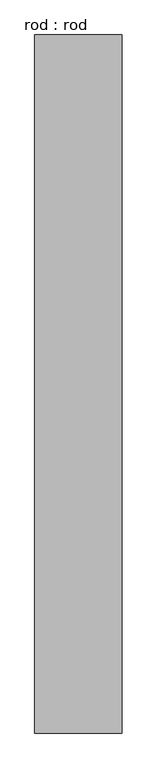
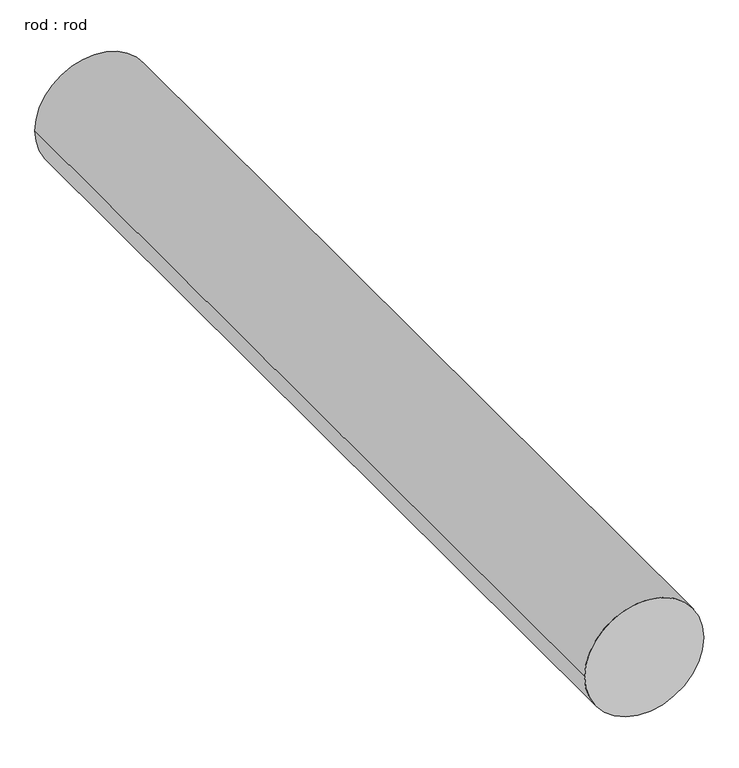
"""IFC4 building model written with IfcOpenShell, lengths in millimetres: proxy geometry, rod : rod."""

from ifc_helpers import new_model, si_unit, point, frame, frame_2d, origin, place, context, project, spatial, circle_curve, trimmed, segment, composite_curve, outline, extrude, source, transform, mapped, element, save


def rod_rod_60906cfb(model_context):
    return source(origin(), model_context, "Body", "SweptSolid", [
        extrude(outline(composite_curve([segment(trimmed(circle_curve(frame_2d((0.0108462, 0.0)), 200.0), [point((0.0108462, 200.0))], [point((0.0108462, -200.0))], False, "CARTESIAN"), True, "CONTINUOUS"), segment(trimmed(circle_curve(frame_2d((0.0108462, 0.0)), 200.0), [point((0.0108462, -200.0))], [point((0.0108462, 200.0))], False, "CARTESIAN"), True, "CONTINUOUS")], self_intersect=False)), frame((0.0, 2492.7286153, 0.0), z_axis=(0.0, 1.0, 0.0), x_axis=(0.0, 0.0, 1.0)), (0.0, 0.0, 1.0), 3200.0),
    ])


if __name__ == "__main__":
    model = new_model("IFC4")
    model_context = context("Model", 3, world=origin())
    ifc_project = project(units=[si_unit("LENGTHUNIT", "METRE", prefix="MILLI")], contexts=[model_context])
    site = spatial("IfcSite", under=ifc_project)
    building = spatial("IfcBuilding", under=site)
    placement = place(None, origin())
    rod_rod_shape = rod_rod_60906cfb(model_context)
    element("IfcBuildingElementProxy", 1, Name="rod : rod", ObjectType="rod : rod", at=placement, inside=building, context=model_context, shape_type="MappedRepresentation", body=[
        mapped(rod_rod_shape, transform((0.0, 0.0, 0.0), x_axis=(1.0, 0.0, 0.0), y_axis=(0.0, 1.0, 0.0), z_axis=(0.0, 0.0, 1.0))),
    ])
    save(model, "model.ifc")

# Revit data of these elements
# Type "rod : rod"
#   Default Elevation = 0
